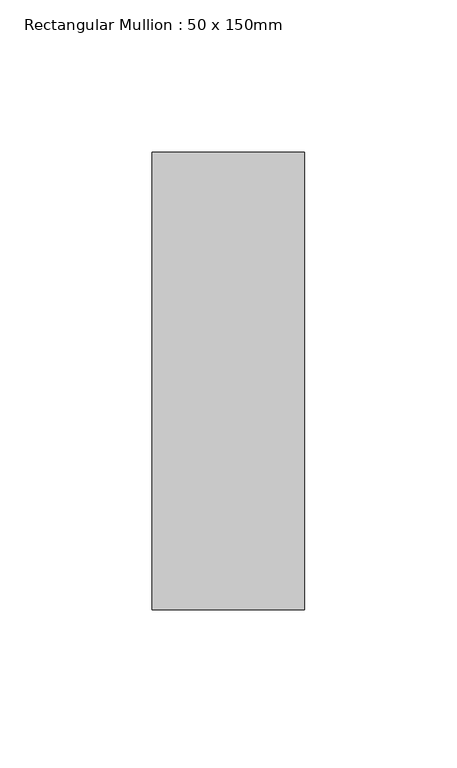
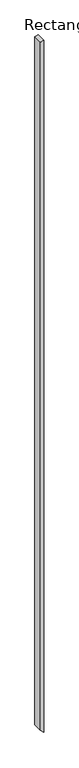
"""IFC4 building model written with IfcOpenShell, lengths in millimetres: member geometry, Rectangular Mullion : 50 x 150mm."""

from ifc_helpers import new_model, si_unit, frame, origin, place, context, project, spatial, polyline, outline, extrude, source, transform, mapped, element, save


def rectangular_mullion_50_x_150mm_985ce2fd(model_context):
    return source(origin(), model_context, "Body", "SweptSolid", [
        extrude(outline(polyline([(0.0, 0.0), (-11.7200342, -50.0), (-11395.4612493, -50.0), (-11440.3058664, 0.0), (0.0, 0.0)])), frame((0.0, -75.0, 0.0), z_axis=(0.0, 1.0, 0.0), x_axis=(0.0, 0.0, 1.0)), (0.0, 0.0, 1.0), 150.0),
    ])


if __name__ == "__main__":
    model = new_model("IFC4")
    model_context = context("Model", 3, world=origin())
    ifc_project = project(units=[si_unit("LENGTHUNIT", "METRE", prefix="MILLI")], contexts=[model_context])
    site = spatial("IfcSite", under=ifc_project)
    building = spatial("IfcBuilding", under=site)
    placement = place(None, origin())
    rectangular_mullion_50_x_150mm_shape = rectangular_mullion_50_x_150mm_985ce2fd(model_context)
    element("IfcMember", 1, ObjectType="Rectangular Mullion : 50 x 150mm", at=placement, inside=building, context=model_context, shape_type="MappedRepresentation", body=[
        mapped(rectangular_mullion_50_x_150mm_shape, transform((0.0, 0.0, 0.0), x_axis=(1.0, 0.0, 0.0), y_axis=(0.0, 1.0, 0.0), z_axis=(0.0, 0.0, 1.0))),
    ])
    save(model, "model.ifc")

# Revit data of these elements
# Type "Rectangular Mullion : 50 x 150mm"
#   built-in parameter 1007304 = 0.492126 (stored number, unit not read)
#   built-in parameter 1007301 = 0.082021 (stored number, unit not read)
#   built-in parameter 1007300 = 0.082021 (stored number, unit not read)
# Element 1 (IfcMember, "Rectangular Mullion : 50 x 150mm")
#   Materials on its faces: "Metal - Aluminium"
# Materials
#   "Metal - Aluminium": class "Metal", colour RGB 247 247 247, transparency 0
